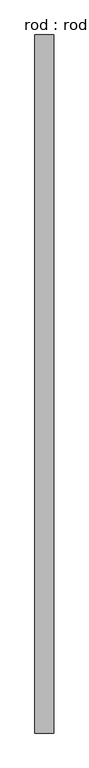
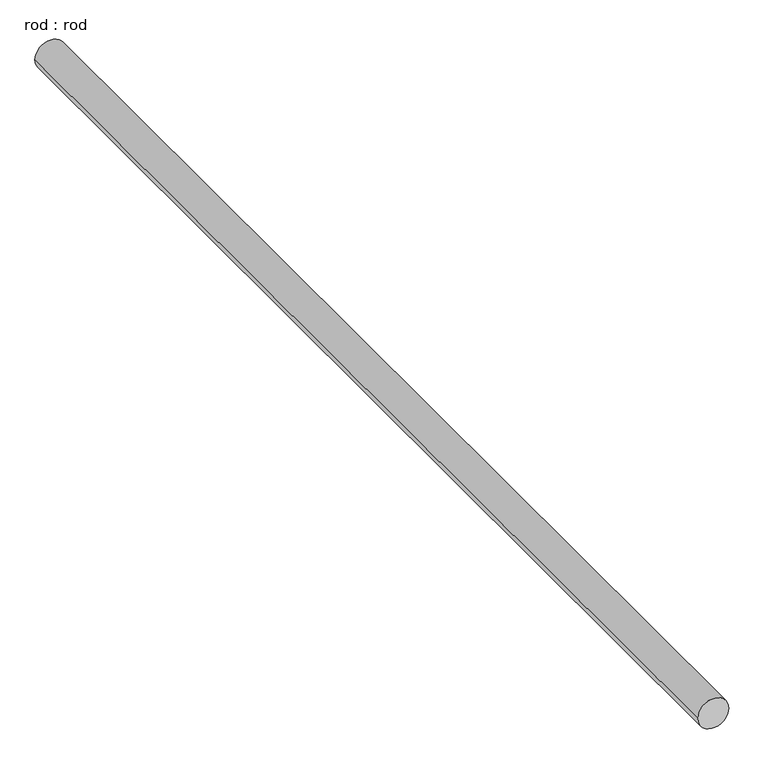
"""IFC4 building model written with IfcOpenShell, lengths in millimetres: proxy geometry, rod : rod."""

import ifcopenshell
import ifcopenshell.guid

model = None  # the IFC model being written
_history = None  # IfcOwnerHistory: only IFC2X3 demands one
_inside = {}  # id of a spatial element -> (the spatial element, [elements in it])
_under = {}  # id of a project, library or spatial element -> (it, [spatial elements below it])
_declared = {}  # id of a project -> (the project, [libraries it declares])
_typed = {}  # id of a type object -> (the type object, [elements of that type])
_made_of = {}  # id of a material, layer set ... -> (it, [elements and type objects made of it])


def new_model(schema):
    """Start an empty IFC model of exactly this schema.

    Asked for "IFC4X3", IfcOpenShell would pick the latest addendum, in which some entities
    have other attributes; the version numbers below select the first issue.
    IFC2X3 requires an IfcOwnerHistory on every rooted entity: one is made here for all.
    """
    global model, _history
    if schema == "IFC4X3":
        model = ifcopenshell.file(schema_version=(4, 3, 0, 0))
    else:
        model = ifcopenshell.file(schema=schema)
    _inside.clear()
    _under.clear()
    _declared.clear()
    _typed.clear()
    _made_of.clear()
    _history = None
    if model.schema == "IFC2X3":
        org = make("IfcOrganization", Name="unknown")
        user = make(
            "IfcPersonAndOrganization",
            ThePerson=make("IfcPerson", FamilyName="unknown"),
            TheOrganization=org,
        )
        app = make(
            "IfcApplication",
            ApplicationDeveloper=org,
            Version="unknown",
            ApplicationFullName="unknown",
            ApplicationIdentifier="unknown",
        )
        _history = make(
            "IfcOwnerHistory",
            OwningUser=user,
            OwningApplication=app,
            ChangeAction="ADDED",
            CreationDate=0,
        )
    return model


def make(cls, **values):
    """One entity of the class cls with the attributes given. An attribute that is None is left unset."""
    return model.create_entity(
        cls, **{name: value for name, value in values.items() if value is not None}
    )


def rooted(cls, **values):
    """An entity with a GlobalId (a new one), such as an element, a storey or a relation."""
    return make(cls, GlobalId=ifcopenshell.guid.new(), OwnerHistory=_history, **values)


def si_unit(unit_type, name, prefix=None):
    """IfcSIUnit, for example si_unit("LENGTHUNIT", "METRE", prefix="MILLI")."""
    return make("IfcSIUnit", UnitType=unit_type, Prefix=prefix, Name=name)


def assignment(units):
    """IfcUnitAssignment: the units of a project."""
    return None if units is None else make("IfcUnitAssignment", Units=units)


def point(xyz):
    """IfcCartesianPoint."""
    return None if xyz is None else make("IfcCartesianPoint", Coordinates=xyz)


def direction(xyz):
    """IfcDirection."""
    return None if xyz is None else make("IfcDirection", DirectionRatios=xyz)


def frame(location, z_axis=None, x_axis=None):
    """IfcAxis2Placement3D, a coordinate frame: its origin and axes. An axis left out is left unset."""
    return make(
        "IfcAxis2Placement3D",
        Location=point(location),
        Axis=direction(z_axis),
        RefDirection=direction(x_axis),
    )


def frame_2d(location, x_axis=None):
    """IfcAxis2Placement2D, a coordinate frame in the plane: its origin and x axis."""
    return make(
        "IfcAxis2Placement2D", Location=point(location), RefDirection=direction(x_axis)
    )


def origin():
    """The frame at (0, 0, 0) with its axes left unset."""
    return frame((0.0, 0.0, 0.0))


def place(relative_to, where):
    """IfcLocalPlacement: puts the frame where relative to a parent placement (None: the world)."""
    return make(
        "IfcLocalPlacement", PlacementRelTo=relative_to, RelativePlacement=where
    )


def context(
    kind, dimensions, precision=None, world=None, true_north=None, identifier=None
):
    """IfcGeometricRepresentationContext, for example the 3D "Model" context."""
    return make(
        "IfcGeometricRepresentationContext",
        ContextIdentifier=identifier,
        ContextType=kind,
        CoordinateSpaceDimension=dimensions,
        Precision=precision,
        WorldCoordinateSystem=world,
        TrueNorth=true_north,
    )


def project(units=None, contexts=None):
    """IfcProject with its units and contexts."""
    return rooted(
        "IfcProject",
        Name="project",
        RepresentationContexts=contexts,
        UnitsInContext=assignment(units),
    )


def spatial(cls, under=None, at=None, **own):
    """A site, building, storey or space (cls), placed at a placement, below another one or the project."""
    s = rooted(cls, ObjectPlacement=at, **own)
    if under is not None:
        _under.setdefault(under.id(), (under, []))[1].append(s)
    return s


def circle_curve(where, radius):
    """IfcCircle in the frame where."""
    return make("IfcCircle", Position=where, Radius=radius)


def trimmed(basis, trim1, trim2, sense, master):
    """IfcTrimmedCurve: the piece of a basis curve between two trims."""
    return make(
        "IfcTrimmedCurve",
        BasisCurve=basis,
        Trim1=trim1,
        Trim2=trim2,
        SenseAgreement=sense,
        MasterRepresentation=master,
    )


def segment(curve, same_sense, transition):
    """IfcCompositeCurveSegment."""
    return make(
        "IfcCompositeCurveSegment",
        Transition=transition,
        SameSense=same_sense,
        ParentCurve=curve,
    )


def composite_curve(segments, self_intersect=None):
    """IfcCompositeCurve: segments joined end to end."""
    return make("IfcCompositeCurve", Segments=segments, SelfIntersect=self_intersect)


def outline(outer, holes=None, kind="AREA"):
    """IfcArbitraryClosedProfileDef: a profile drawn as a closed curve; with holes, ...WithVoids."""
    if holes is None:
        return make("IfcArbitraryClosedProfileDef", ProfileType=kind, OuterCurve=outer)
    return make(
        "IfcArbitraryProfileDefWithVoids",
        ProfileType=kind,
        OuterCurve=outer,
        InnerCurves=holes,
    )


def extrude(swept, where, along, depth):
    """IfcExtrudedAreaSolid: the profile swept, set in the frame where, extruded along a direction by depth."""
    return make(
        "IfcExtrudedAreaSolid",
        SweptArea=swept,
        Position=where,
        ExtrudedDirection=direction(along),
        Depth=depth,
    )


def shape(context_of_items, identifier, shape_type, items):
    """IfcShapeRepresentation: the items that make up one representation, for example the "Body"."""
    return make(
        "IfcShapeRepresentation",
        ContextOfItems=context_of_items,
        RepresentationIdentifier=identifier,
        RepresentationType=shape_type,
        Items=items,
    )


def source(mapping_origin, context_of_items, identifier, shape_type, items):
    """IfcRepresentationMap: a shape defined once, which mapped items show again and again."""
    return make(
        "IfcRepresentationMap",
        MappingOrigin=mapping_origin,
        MappedRepresentation=shape(context_of_items, identifier, shape_type, items),
    )


def transform(
    local_origin,
    x_axis=None,
    y_axis=None,
    z_axis=None,
    scale=None,
    scale2=None,
    scale3=None,
    uniform=True,
):
    """IfcCartesianTransformationOperator3D, or its non-uniform kind. x_axis, y_axis, z_axis: its Axis1, 2, 3."""
    if uniform:
        return make(
            "IfcCartesianTransformationOperator3D",
            Axis1=direction(x_axis),
            Axis2=direction(y_axis),
            LocalOrigin=point(local_origin),
            Scale=scale,
            Axis3=direction(z_axis),
        )
    return make(
        "IfcCartesianTransformationOperator3DnonUniform",
        Axis1=direction(x_axis),
        Axis2=direction(y_axis),
        LocalOrigin=point(local_origin),
        Scale=scale,
        Axis3=direction(z_axis),
        Scale2=scale2,
        Scale3=scale3,
    )


def mapped(mapping_source, mapping_target):
    """IfcMappedItem: shows the shape of a source again, moved by a transform."""
    return make(
        "IfcMappedItem", MappingSource=mapping_source, MappingTarget=mapping_target
    )


def made_of(thing, what):
    """Note that an element or type object is made of a material, layer set ...; save() writes the relation."""
    if what is not None:
        _made_of.setdefault(what.id(), (what, []))[1].append(thing)
    return thing


def element(
    cls,
    number,
    at=None,
    inside=None,
    cuts=None,
    type_object=None,
    material=None,
    context=None,
    identifier="Body",
    shape_type=None,
    held_by="IfcProductDefinitionShape",
    body=None,
    shapes=None,
    **own,
):
    """One element of the class cls, such as IfcWall. Its Tag is "e" and its number.

    at: its placement. inside: the storey or other place that contains it. cuts: it is an
    opening in that element (IfcRelVoidsElement). A single representation is given by context,
    identifier, shape_type and body (its items); several are given by shapes. held_by: the class
    of the entity that holds the representations. save() writes the other relations.
    """
    e = rooted(cls, Tag="e%d" % number, ObjectPlacement=at, **own)
    if body is not None:
        shapes = [shape(context, identifier, shape_type, body)]
    if shapes is not None:
        e.Representation = make(held_by, Representations=shapes)
    if inside is not None:
        _inside.setdefault(inside.id(), (inside, []))[1].append(e)
    if cuts is not None:
        rooted(
            "IfcRelVoidsElement", RelatingBuildingElement=cuts, RelatedOpeningElement=e
        )
    if type_object is not None:
        _typed.setdefault(type_object.id(), (type_object, []))[1].append(e)
    return made_of(e, material)


def aggregate(whole, parts):
    """IfcRelAggregates: a whole, such as a stair, and the parts it consists of."""
    return rooted("IfcRelAggregates", RelatingObject=whole, RelatedObjects=parts)


def save(model, path):
    """Write the relations noted so far, then the file.

    IfcRelAggregates (storeys below a building ...), IfcRelContainedInSpatialStructure (elements
    in a storey), IfcRelDefinesByType, IfcRelAssociatesMaterial and IfcRelDeclares: one each for
    every whole, place, type object, material and project.
    """
    for whole, parts in _under.values():
        aggregate(whole, parts)
    for where, things in _inside.values():
        rooted(
            "IfcRelContainedInSpatialStructure",
            RelatedElements=things,
            RelatingStructure=where,
        )
    for kind, things in _typed.values():
        rooted("IfcRelDefinesByType", RelatedObjects=things, RelatingType=kind)
    for what, things in _made_of.values():
        rooted("IfcRelAssociatesMaterial", RelatedObjects=things, RelatingMaterial=what)
    for by, libraries in _declared.values():
        rooted("IfcRelDeclares", RelatingContext=by, RelatedDefinitions=libraries)
    model.write(path)


def rod_rod_35d76520(model_context):
    return source(origin(), model_context, "Body", "SweptSolid", [
        extrude(outline(composite_curve([segment(trimmed(circle_curve(frame_2d((0.0108462, 0.0)), 200.0), [point((0.0108462, 200.0))], [point((0.0108462, -200.0))], False, "CARTESIAN"), True, "CONTINUOUS"), segment(trimmed(circle_curve(frame_2d((0.0108462, 0.0)), 200.0), [point((0.0108462, -200.0))], [point((0.0108462, 200.0))], False, "CARTESIAN"), True, "CONTINUOUS")], self_intersect=False)), frame((0.0, -3296.9822749, 0.0), z_axis=(0.0, 1.0, 0.0), x_axis=(0.0, 0.0, 1.0)), (0.0, 0.0, 1.0), 14779.4217804),
    ])


if __name__ == "__main__":
    model = new_model("IFC4")
    model_context = context("Model", 3, world=origin())
    ifc_project = project(units=[si_unit("LENGTHUNIT", "METRE", prefix="MILLI")], contexts=[model_context])
    site = spatial("IfcSite", under=ifc_project)
    building = spatial("IfcBuilding", under=site)
    placement = place(None, origin())
    rod_rod_shape = rod_rod_35d76520(model_context)
    element("IfcBuildingElementProxy", 1, Name="rod : rod", ObjectType="rod : rod", at=placement, inside=building, context=model_context, shape_type="MappedRepresentation", body=[
        mapped(rod_rod_shape, transform((0.0, 0.0, 0.0), x_axis=(1.0, 0.0, 0.0), y_axis=(0.0, 1.0, 0.0), z_axis=(0.0, 0.0, 1.0))),
    ])
    save(model, "model.ifc")

# Revit data of these elements
# Type "rod : rod"
#   Default Elevation = 0
